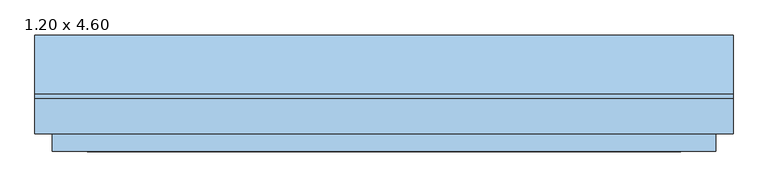
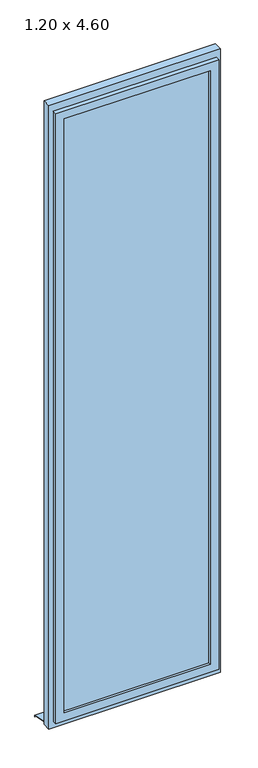
"""IFC4 building model written with IfcOpenShell, lengths in millimetres: window geometry, Fenstertür 1-flg : 1.20 x 4.60."""

from ifc_helpers import new_model, si_unit, frame, origin, place, context, project, spatial, polyline, outline, extrude, faceted_brep, source, transform, mapped, element, save


def window_1_20_x_4_60_7575aed5(model_context):
    return source(origin(), model_context, "Body", "SolidModel", [
        extrude(outline(polyline([(4600.0, 600.0), (4600.0, -600.0), (0.0, -600.0), (0.0, 600.0), (4600.0, 600.0)]), holes=[polyline([(4520.0, 540.0), (80.0, 540.0), (80.0, -540.0), (4520.0, -540.0), (4520.0, 540.0)])]), frame((0.0, -80.0, 0.0), z_axis=(0.0, 1.0, 0.0), x_axis=(0.0, 0.0, 1.0)), (0.0, 0.0, 1.0), 60.0),
        faceted_brep([(570.0, -80.0, 4550.0), (570.0, -110.0, 4550.0), (570.0, -110.0, 50.0), (570.0, -80.0, 50.0), (-570.0, -110.0, 4550.0), (-570.0, -110.0, 50.0), (510.0, -110.0, 110.0), (-510.0, -110.0, 110.0), (-510.0, -110.0, 4490.0), (510.0, -110.0, 4490.0), (-570.0, -80.0, 50.0), (-570.0, -80.0, 4550.0), (540.0, -80.0, 4520.0), (-540.0, -80.0, 4520.0), (-540.0, -80.0, 80.0), (540.0, -80.0, 80.0), (540.0, -50.0, 4520.0), (540.0, -50.0, 80.0), (-540.0, -50.0, 80.0), (-540.0, -50.0, 4520.0), (510.0, -50.0, 4490.0), (-510.0, -50.0, 4490.0), (-510.0, -50.0, 110.0), (510.0, -50.0, 110.0)], [[[0, 1, 2, 3]], [[1, 4, 5, 2], [6, 7, 8, 9]], [[3, 2, 5, 10]], [[3, 10, 11, 0], [12, 13, 14, 15]], [[16, 12, 15, 17]], [[17, 15, 14, 18]], [[17, 18, 19, 16], [20, 21, 22, 23]], [[9, 20, 23, 6]], [[6, 23, 22, 7]], [[10, 5, 4, 11]], [[18, 14, 13, 19]], [[7, 22, 21, 8]], [[11, 4, 1, 0]], [[19, 13, 12, 16]], [[8, 21, 20, 9]]]),
        extrude(outline(polyline([(-9.9778457, 20.0), (90.0, 0.0), (90.0, -10.0), (88.0, -10.0), (88.0, -1.6395366), (-10.1759277, 18.0), (-20.0, 18.0), (-20.0, 20.0), (-9.9778457, 20.0)])), frame((-600.0, 0.0, 0.0), z_axis=(1.0, 0.0, 0.0), x_axis=(0.0, 1.0, 0.0)), (0.0, 0.0, 1.0), 1200.0),
        extrude(outline(polyline([(510.0, -95.0), (-510.0, -95.0), (-510.0, -65.0), (510.0, -65.0), (510.0, -95.0)])), frame((0.0, 0.0, 110.0), z_axis=(0.0, 0.0, 1.0), x_axis=(1.0, 0.0, 0.0)), (0.0, 0.0, 1.0), 4380.0),
    ])


if __name__ == "__main__":
    model = new_model("IFC4")
    model_context = context("Model", 3, world=origin())
    ifc_project = project(units=[si_unit("LENGTHUNIT", "METRE", prefix="MILLI")], contexts=[model_context])
    site = spatial("IfcSite", under=ifc_project)
    building = spatial("IfcBuilding", under=site)
    placement = place(None, origin())
    window_1_20_x_4_60_shape = window_1_20_x_4_60_7575aed5(model_context)
    element("IfcWindow", 1, ObjectType="Fenstertür 1-flg : 1.20 x 4.60", at=placement, inside=building, context=model_context, shape_type="MappedRepresentation", body=[
        mapped(window_1_20_x_4_60_shape, transform((0.0, 0.0, 0.0), x_axis=(1.0, 0.0, 0.0), y_axis=(0.0, 1.0, 0.0), z_axis=(0.0, 0.0, 1.0))),
    ])
    save(model, "model.ifc")

# Revit data of these elements
# Type "Fenstertür 1-flg : 1.20 x 4.60"
#   Type Mark = "62"
#   Operation = "SinglePanel"
#   Construction Type Id = "SGL"
#   Keynote = "16.05.01"
#   Analytic Construction = "Große Fenster mit Einfachverglasung"
#   Visual Light Transmittance = 0.9
#   Solar Heat Gain Coefficient = 0.86
#   Rough Width = 1.200 m
#   Rough Height = 4.600 m
#   Heat Transfer Coefficient (U) = 5.5617 W/(m²·K)
#   Rahmentiefe = 0.060 m
#   Rahmenhöhe unten = 0.080 m
#   Höhe oberer  Rahmen = 0.080 m
#   Rahmenbreite = 0.060 m
#   Height = 4.600 m
#   Tiefe Flügel = 0.060 m
#   Flügelbreite = 0.060 m
#   Einbautiefe (von außen) [instance default] = 0.080 m
#   Width = 1.200 m
#   Sichtbarkeit Sturzlinien [instance default] = yes
#   Öffnungsrichtung oben [instance default] = yes
#   Öffnungsrichtung in Draufsicht anzeigen [instance default] = yes
#   Drehflügel 1 [instance default] = yes
#   Bild [instance default] = none
#   Glas [instance default] = none
#   Fensterflügel [instance default] = none
#   Äußere Fensterbank [instance default] = none
#   Wall Closure = (empty or 0)
# Element 1 (IfcWindow, "Fenstertür 1-flg : 1.20 x 4.60")
#   Materials on its faces: "Kunststoff - Weiß", "Glas"
# Materials
#   "Kunststoff - Weiß": class "Kunststoff", colour RGB 249 249 249, transparency 0, Cost = 0
#   "Glas": class "Glas", colour RGB 0 0 255, transparency 0.75, Comments = "Render-Darstellung nicht aktualisiert ", Cost = 0
